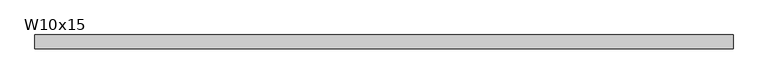
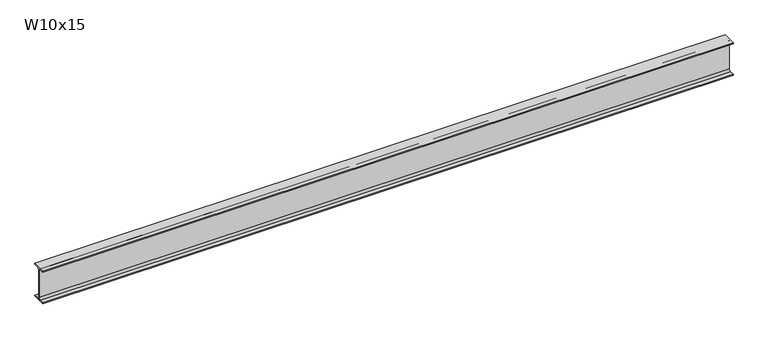
"""IFC4 building model written with IfcOpenShell, lengths in millimetres: beam geometry, RME W-Wide Flange : W10x15."""

from ifc_helpers import new_model, si_unit, point, frame, frame_2d, origin, place, context, project, spatial, polyline, circle_curve, trimmed, segment, composite_curve, outline, extrude, source, transform, mapped, element, save


def w10x15_a1ac2403(model_context):
    return source(origin(), model_context, "Body", "SweptSolid", [
        extrude(outline(composite_curve([segment(polyline([(50.8, -120.142), (50.8, -127.0), (-50.8, -127.0), (-50.8, -120.142), (-16.7005, -120.142)]), True, "CONTINUOUS"), segment(trimmed(circle_curve(frame_2d((-16.7005, -106.3625)), 13.7795), [point((-16.7005, -120.142))], [point((-2.921, -106.3625))], True, "CARTESIAN"), True, "CONTINUOUS"), segment(polyline([(-2.921, -106.3625), (-2.921, 106.3625)]), True, "CONTINUOUS"), segment(trimmed(circle_curve(frame_2d((-16.7005, 106.3625)), 13.7795), [point((-2.921, 106.3625))], [point((-16.7005, 120.142))], True, "CARTESIAN"), True, "CONTINUOUS"), segment(polyline([(-16.7005, 120.142), (-50.8, 120.142), (-50.8, 127.0), (50.8, 127.0), (50.8, 120.142), (16.7005, 120.142)]), True, "CONTINUOUS"), segment(trimmed(circle_curve(frame_2d((16.7005, 106.3625)), 13.7795), [point((16.7005, 120.142))], [point((2.921, 106.3625))], True, "CARTESIAN"), True, "CONTINUOUS"), segment(polyline([(2.921, 106.3625), (2.921, -106.3625)]), True, "CONTINUOUS"), segment(trimmed(circle_curve(frame_2d((16.7005, -106.3625)), 13.7795), [point((2.921, -106.3625))], [point((16.7005, -120.142))], True, "CARTESIAN"), True, "CONTINUOUS"), segment(polyline([(16.7005, -120.142), (50.8, -120.142)]), True, "CONTINUOUS")], self_intersect=False)), frame((-2553.6554804, 0.0, 0.0), z_axis=(1.0, 0.0, 0.0), x_axis=(0.0, 1.0, 0.0)), (0.0, 0.0, 1.0), 5107.3109608),
    ])


if __name__ == "__main__":
    model = new_model("IFC4")
    model_context = context("Model", 3, world=origin())
    ifc_project = project(units=[si_unit("LENGTHUNIT", "METRE", prefix="MILLI")], contexts=[model_context])
    site = spatial("IfcSite", under=ifc_project)
    building = spatial("IfcBuilding", under=site)
    placement = place(None, origin())
    w10x15_shape = w10x15_a1ac2403(model_context)
    element("IfcBeam", 1, ObjectType="RME W-Wide Flange : W10x15", at=placement, inside=building, context=model_context, shape_type="MappedRepresentation", body=[
        mapped(w10x15_shape, transform((0.0, 0.0, 0.0), x_axis=(1.0, 0.0, 0.0), y_axis=(0.0, 1.0, 0.0), z_axis=(0.0, 0.0, 1.0))),
    ])
    save(model, "model.ifc")

# Revit data of these elements
# Type "RME W-Wide Flange : W10x15"
#   WELD P [instance default] = ""
#   WELD LE [instance default] = ""
#   WELD D [instance default] = ""
#   TOP SECTION SIZE [instance default] = ""
#   TOP SECTION LENGTH [instance default] = ""
#   REMARKS [instance default] = ""
#   REINF TYPE [instance default] = ""
#   Nominal Size = "W24"
#   End Bearing Capacity [instance default] = ""
#   BOT SECTION SIZE [instance default] = ""
#   BOT SECTION LENGTH [instance default] = ""
#   Assembly Code = "B10"
#   W = 15
#   Start Extension Calculation [instance default] = 10' - 0"
#   Start Extension [instance default] = -0' - 0 1/2"
#   End Extension Calculation [instance default] = 10' - 0"
#   End Extension [instance default] = -0' - 0 1/2"
#   Length [instance default] = 5' - 0"
#   bf = 0' - 4"
#   d = 0' - 10"
#   k = 0' - 0 13/16"
#   k2 = 0' - 0.5425"
#   tf = 0' - 0.27"
#   tw = 0' - 0.23"
#   A = 0.030625 SF
#   Structural Material [instance default] = Metal - Steel - ASTM A992
# Element 1 (IfcBeam, "RME W-Wide Flange : W10x15")
#   Length = 16' - 9.07523"
#   Materials on its faces: "Metal - Steel - ASTM A992"
# Materials
#   "Metal - Steel - ASTM A992": class "Metal", colour RGB 255 128 0, transparency 0
